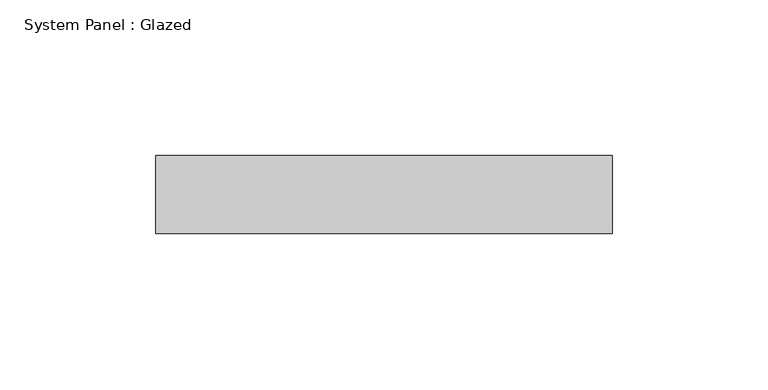
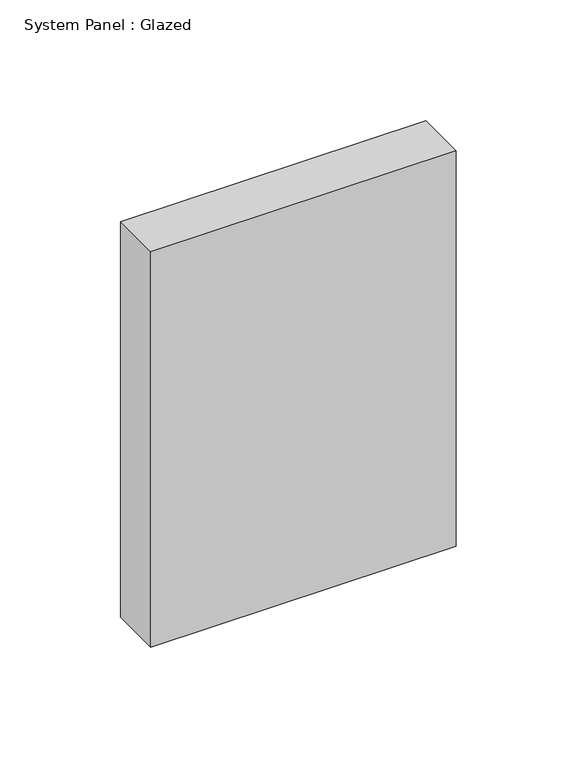
"""IFC4 building model written with IfcOpenShell, lengths in millimetres: plate geometry, System Panel : Glazed."""

import ifcopenshell
import ifcopenshell.guid

model = None  # the IFC model being written
_history = None  # IfcOwnerHistory: only IFC2X3 demands one
_inside = {}  # id of a spatial element -> (the spatial element, [elements in it])
_under = {}  # id of a project, library or spatial element -> (it, [spatial elements below it])
_declared = {}  # id of a project -> (the project, [libraries it declares])
_typed = {}  # id of a type object -> (the type object, [elements of that type])
_made_of = {}  # id of a material, layer set ... -> (it, [elements and type objects made of it])


def new_model(schema):
    """Start an empty IFC model of exactly this schema.

    Asked for "IFC4X3", IfcOpenShell would pick the latest addendum, in which some entities
    have other attributes; the version numbers below select the first issue.
    IFC2X3 requires an IfcOwnerHistory on every rooted entity: one is made here for all.
    """
    global model, _history
    if schema == "IFC4X3":
        model = ifcopenshell.file(schema_version=(4, 3, 0, 0))
    else:
        model = ifcopenshell.file(schema=schema)
    _inside.clear()
    _under.clear()
    _declared.clear()
    _typed.clear()
    _made_of.clear()
    _history = None
    if model.schema == "IFC2X3":
        org = make("IfcOrganization", Name="unknown")
        user = make(
            "IfcPersonAndOrganization",
            ThePerson=make("IfcPerson", FamilyName="unknown"),
            TheOrganization=org,
        )
        app = make(
            "IfcApplication",
            ApplicationDeveloper=org,
            Version="unknown",
            ApplicationFullName="unknown",
            ApplicationIdentifier="unknown",
        )
        _history = make(
            "IfcOwnerHistory",
            OwningUser=user,
            OwningApplication=app,
            ChangeAction="ADDED",
            CreationDate=0,
        )
    return model


def make(cls, **values):
    """One entity of the class cls with the attributes given. An attribute that is None is left unset."""
    return model.create_entity(
        cls, **{name: value for name, value in values.items() if value is not None}
    )


def rooted(cls, **values):
    """An entity with a GlobalId (a new one), such as an element, a storey or a relation."""
    return make(cls, GlobalId=ifcopenshell.guid.new(), OwnerHistory=_history, **values)


def si_unit(unit_type, name, prefix=None):
    """IfcSIUnit, for example si_unit("LENGTHUNIT", "METRE", prefix="MILLI")."""
    return make("IfcSIUnit", UnitType=unit_type, Prefix=prefix, Name=name)


def assignment(units):
    """IfcUnitAssignment: the units of a project."""
    return None if units is None else make("IfcUnitAssignment", Units=units)


def point(xyz):
    """IfcCartesianPoint."""
    return None if xyz is None else make("IfcCartesianPoint", Coordinates=xyz)


def direction(xyz):
    """IfcDirection."""
    return None if xyz is None else make("IfcDirection", DirectionRatios=xyz)


def frame(location, z_axis=None, x_axis=None):
    """IfcAxis2Placement3D, a coordinate frame: its origin and axes. An axis left out is left unset."""
    return make(
        "IfcAxis2Placement3D",
        Location=point(location),
        Axis=direction(z_axis),
        RefDirection=direction(x_axis),
    )


def origin():
    """The frame at (0, 0, 0) with its axes left unset."""
    return frame((0.0, 0.0, 0.0))


def origin_with_axes():
    """The frame at (0, 0, 0) with the z axis (0, 0, 1) and the x axis (1, 0, 0) written out."""
    return frame((0.0, 0.0, 0.0), z_axis=(0.0, 0.0, 1.0), x_axis=(1.0, 0.0, 0.0))


def place(relative_to, where):
    """IfcLocalPlacement: puts the frame where relative to a parent placement (None: the world)."""
    return make(
        "IfcLocalPlacement", PlacementRelTo=relative_to, RelativePlacement=where
    )


def context(
    kind, dimensions, precision=None, world=None, true_north=None, identifier=None
):
    """IfcGeometricRepresentationContext, for example the 3D "Model" context."""
    return make(
        "IfcGeometricRepresentationContext",
        ContextIdentifier=identifier,
        ContextType=kind,
        CoordinateSpaceDimension=dimensions,
        Precision=precision,
        WorldCoordinateSystem=world,
        TrueNorth=true_north,
    )


def project(units=None, contexts=None):
    """IfcProject with its units and contexts."""
    return rooted(
        "IfcProject",
        Name="project",
        RepresentationContexts=contexts,
        UnitsInContext=assignment(units),
    )


def spatial(cls, under=None, at=None, **own):
    """A site, building, storey or space (cls), placed at a placement, below another one or the project."""
    s = rooted(cls, ObjectPlacement=at, **own)
    if under is not None:
        _under.setdefault(under.id(), (under, []))[1].append(s)
    return s


def polyline(points):
    """IfcPolyline through the points."""
    return make("IfcPolyline", Points=[point(p) for p in points])


def outline(outer, holes=None, kind="AREA"):
    """IfcArbitraryClosedProfileDef: a profile drawn as a closed curve; with holes, ...WithVoids."""
    if holes is None:
        return make("IfcArbitraryClosedProfileDef", ProfileType=kind, OuterCurve=outer)
    return make(
        "IfcArbitraryProfileDefWithVoids",
        ProfileType=kind,
        OuterCurve=outer,
        InnerCurves=holes,
    )


def extrude(swept, where, along, depth):
    """IfcExtrudedAreaSolid: the profile swept, set in the frame where, extruded along a direction by depth."""
    return make(
        "IfcExtrudedAreaSolid",
        SweptArea=swept,
        Position=where,
        ExtrudedDirection=direction(along),
        Depth=depth,
    )


def shape(context_of_items, identifier, shape_type, items):
    """IfcShapeRepresentation: the items that make up one representation, for example the "Body"."""
    return make(
        "IfcShapeRepresentation",
        ContextOfItems=context_of_items,
        RepresentationIdentifier=identifier,
        RepresentationType=shape_type,
        Items=items,
    )


def source(mapping_origin, context_of_items, identifier, shape_type, items):
    """IfcRepresentationMap: a shape defined once, which mapped items show again and again."""
    return make(
        "IfcRepresentationMap",
        MappingOrigin=mapping_origin,
        MappedRepresentation=shape(context_of_items, identifier, shape_type, items),
    )


def transform(
    local_origin,
    x_axis=None,
    y_axis=None,
    z_axis=None,
    scale=None,
    scale2=None,
    scale3=None,
    uniform=True,
):
    """IfcCartesianTransformationOperator3D, or its non-uniform kind. x_axis, y_axis, z_axis: its Axis1, 2, 3."""
    if uniform:
        return make(
            "IfcCartesianTransformationOperator3D",
            Axis1=direction(x_axis),
            Axis2=direction(y_axis),
            LocalOrigin=point(local_origin),
            Scale=scale,
            Axis3=direction(z_axis),
        )
    return make(
        "IfcCartesianTransformationOperator3DnonUniform",
        Axis1=direction(x_axis),
        Axis2=direction(y_axis),
        LocalOrigin=point(local_origin),
        Scale=scale,
        Axis3=direction(z_axis),
        Scale2=scale2,
        Scale3=scale3,
    )


def mapped(mapping_source, mapping_target):
    """IfcMappedItem: shows the shape of a source again, moved by a transform."""
    return make(
        "IfcMappedItem", MappingSource=mapping_source, MappingTarget=mapping_target
    )


def made_of(thing, what):
    """Note that an element or type object is made of a material, layer set ...; save() writes the relation."""
    if what is not None:
        _made_of.setdefault(what.id(), (what, []))[1].append(thing)
    return thing


def element(
    cls,
    number,
    at=None,
    inside=None,
    cuts=None,
    type_object=None,
    material=None,
    context=None,
    identifier="Body",
    shape_type=None,
    held_by="IfcProductDefinitionShape",
    body=None,
    shapes=None,
    **own,
):
    """One element of the class cls, such as IfcWall. Its Tag is "e" and its number.

    at: its placement. inside: the storey or other place that contains it. cuts: it is an
    opening in that element (IfcRelVoidsElement). A single representation is given by context,
    identifier, shape_type and body (its items); several are given by shapes. held_by: the class
    of the entity that holds the representations. save() writes the other relations.
    """
    e = rooted(cls, Tag="e%d" % number, ObjectPlacement=at, **own)
    if body is not None:
        shapes = [shape(context, identifier, shape_type, body)]
    if shapes is not None:
        e.Representation = make(held_by, Representations=shapes)
    if inside is not None:
        _inside.setdefault(inside.id(), (inside, []))[1].append(e)
    if cuts is not None:
        rooted(
            "IfcRelVoidsElement", RelatingBuildingElement=cuts, RelatedOpeningElement=e
        )
    if type_object is not None:
        _typed.setdefault(type_object.id(), (type_object, []))[1].append(e)
    return made_of(e, material)


def aggregate(whole, parts):
    """IfcRelAggregates: a whole, such as a stair, and the parts it consists of."""
    return rooted("IfcRelAggregates", RelatingObject=whole, RelatedObjects=parts)


def save(model, path):
    """Write the relations noted so far, then the file.

    IfcRelAggregates (storeys below a building ...), IfcRelContainedInSpatialStructure (elements
    in a storey), IfcRelDefinesByType, IfcRelAssociatesMaterial and IfcRelDeclares: one each for
    every whole, place, type object, material and project.
    """
    for whole, parts in _under.values():
        aggregate(whole, parts)
    for where, things in _inside.values():
        rooted(
            "IfcRelContainedInSpatialStructure",
            RelatedElements=things,
            RelatingStructure=where,
        )
    for kind, things in _typed.values():
        rooted("IfcRelDefinesByType", RelatedObjects=things, RelatingType=kind)
    for what, things in _made_of.values():
        rooted("IfcRelAssociatesMaterial", RelatedObjects=things, RelatingMaterial=what)
    for by, libraries in _declared.values():
        rooted("IfcRelDeclares", RelatingContext=by, RelatedDefinitions=libraries)
    model.write(path)


def system_panel_glazed_44cc28f0(model_context):
    return source(origin(), model_context, "Body", "SweptSolid", [
        extrude(outline(polyline([(73.0866293, 24.5), (-73.0866293, 24.5), (-73.0866293, 49.5), (73.0866293, 49.5), (73.0866293, 24.5)])), origin_with_axes(), (0.0, 0.0, 1.0), 200.0),
    ])


if __name__ == "__main__":
    model = new_model("IFC4")
    model_context = context("Model", 3, world=origin())
    ifc_project = project(units=[si_unit("LENGTHUNIT", "METRE", prefix="MILLI")], contexts=[model_context])
    site = spatial("IfcSite", under=ifc_project)
    building = spatial("IfcBuilding", under=site)
    placement = place(None, origin())
    system_panel_glazed_shape = system_panel_glazed_44cc28f0(model_context)
    element("IfcPlate", 1, ObjectType="System Panel : Glazed", at=placement, inside=building, context=model_context, shape_type="MappedRepresentation", body=[
        mapped(system_panel_glazed_shape, transform((0.0, 0.0, 0.0), x_axis=(1.0, 0.0, 0.0), y_axis=(0.0, 1.0, 0.0), z_axis=(0.0, 0.0, 1.0))),
    ])
    save(model, "model.ifc")

# Revit data of these elements
# Element 1 (IfcPlate, "System Panel : Glazed")
#   Materials on its faces: "Glass"
# Materials
#   "Glass": class "Glass", colour RGB 218 227 224, transparency 0.85, Description = "Soda Lime Glass", Cost = 0
